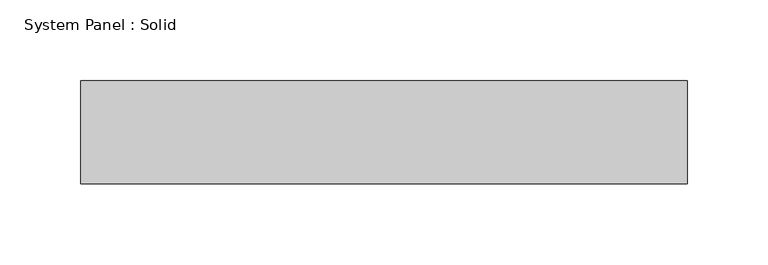
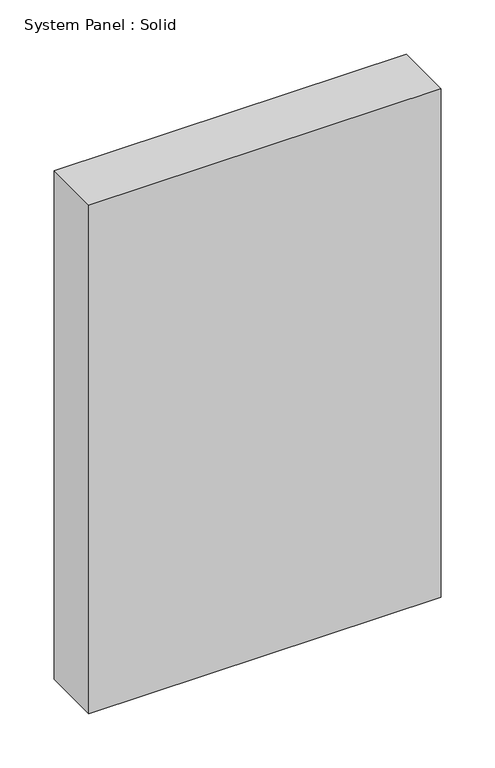
"""IFC4 building model written with IfcOpenShell, lengths in millimetres: plate geometry, System Panel : Solid."""

import ifcopenshell
import ifcopenshell.guid

model = None  # the IFC model being written
_history = None  # IfcOwnerHistory: only IFC2X3 demands one
_inside = {}  # id of a spatial element -> (the spatial element, [elements in it])
_under = {}  # id of a project, library or spatial element -> (it, [spatial elements below it])
_declared = {}  # id of a project -> (the project, [libraries it declares])
_typed = {}  # id of a type object -> (the type object, [elements of that type])
_made_of = {}  # id of a material, layer set ... -> (it, [elements and type objects made of it])


def new_model(schema):
    """Start an empty IFC model of exactly this schema.

    Asked for "IFC4X3", IfcOpenShell would pick the latest addendum, in which some entities
    have other attributes; the version numbers below select the first issue.
    IFC2X3 requires an IfcOwnerHistory on every rooted entity: one is made here for all.
    """
    global model, _history
    if schema == "IFC4X3":
        model = ifcopenshell.file(schema_version=(4, 3, 0, 0))
    else:
        model = ifcopenshell.file(schema=schema)
    _inside.clear()
    _under.clear()
    _declared.clear()
    _typed.clear()
    _made_of.clear()
    _history = None
    if model.schema == "IFC2X3":
        org = make("IfcOrganization", Name="unknown")
        user = make(
            "IfcPersonAndOrganization",
            ThePerson=make("IfcPerson", FamilyName="unknown"),
            TheOrganization=org,
        )
        app = make(
            "IfcApplication",
            ApplicationDeveloper=org,
            Version="unknown",
            ApplicationFullName="unknown",
            ApplicationIdentifier="unknown",
        )
        _history = make(
            "IfcOwnerHistory",
            OwningUser=user,
            OwningApplication=app,
            ChangeAction="ADDED",
            CreationDate=0,
        )
    return model


def make(cls, **values):
    """One entity of the class cls with the attributes given. An attribute that is None is left unset."""
    return model.create_entity(
        cls, **{name: value for name, value in values.items() if value is not None}
    )


def rooted(cls, **values):
    """An entity with a GlobalId (a new one), such as an element, a storey or a relation."""
    return make(cls, GlobalId=ifcopenshell.guid.new(), OwnerHistory=_history, **values)


def si_unit(unit_type, name, prefix=None):
    """IfcSIUnit, for example si_unit("LENGTHUNIT", "METRE", prefix="MILLI")."""
    return make("IfcSIUnit", UnitType=unit_type, Prefix=prefix, Name=name)


def assignment(units):
    """IfcUnitAssignment: the units of a project."""
    return None if units is None else make("IfcUnitAssignment", Units=units)


def point(xyz):
    """IfcCartesianPoint."""
    return None if xyz is None else make("IfcCartesianPoint", Coordinates=xyz)


def direction(xyz):
    """IfcDirection."""
    return None if xyz is None else make("IfcDirection", DirectionRatios=xyz)


def frame(location, z_axis=None, x_axis=None):
    """IfcAxis2Placement3D, a coordinate frame: its origin and axes. An axis left out is left unset."""
    return make(
        "IfcAxis2Placement3D",
        Location=point(location),
        Axis=direction(z_axis),
        RefDirection=direction(x_axis),
    )


def origin():
    """The frame at (0, 0, 0) with its axes left unset."""
    return frame((0.0, 0.0, 0.0))


def origin_with_axes():
    """The frame at (0, 0, 0) with the z axis (0, 0, 1) and the x axis (1, 0, 0) written out."""
    return frame((0.0, 0.0, 0.0), z_axis=(0.0, 0.0, 1.0), x_axis=(1.0, 0.0, 0.0))


def place(relative_to, where):
    """IfcLocalPlacement: puts the frame where relative to a parent placement (None: the world)."""
    return make(
        "IfcLocalPlacement", PlacementRelTo=relative_to, RelativePlacement=where
    )


def context(
    kind, dimensions, precision=None, world=None, true_north=None, identifier=None
):
    """IfcGeometricRepresentationContext, for example the 3D "Model" context."""
    return make(
        "IfcGeometricRepresentationContext",
        ContextIdentifier=identifier,
        ContextType=kind,
        CoordinateSpaceDimension=dimensions,
        Precision=precision,
        WorldCoordinateSystem=world,
        TrueNorth=true_north,
    )


def project(units=None, contexts=None):
    """IfcProject with its units and contexts."""
    return rooted(
        "IfcProject",
        Name="project",
        RepresentationContexts=contexts,
        UnitsInContext=assignment(units),
    )


def spatial(cls, under=None, at=None, **own):
    """A site, building, storey or space (cls), placed at a placement, below another one or the project."""
    s = rooted(cls, ObjectPlacement=at, **own)
    if under is not None:
        _under.setdefault(under.id(), (under, []))[1].append(s)
    return s


def polyline(points):
    """IfcPolyline through the points."""
    return make("IfcPolyline", Points=[point(p) for p in points])


def outline(outer, holes=None, kind="AREA"):
    """IfcArbitraryClosedProfileDef: a profile drawn as a closed curve; with holes, ...WithVoids."""
    if holes is None:
        return make("IfcArbitraryClosedProfileDef", ProfileType=kind, OuterCurve=outer)
    return make(
        "IfcArbitraryProfileDefWithVoids",
        ProfileType=kind,
        OuterCurve=outer,
        InnerCurves=holes,
    )


def extrude(swept, where, along, depth):
    """IfcExtrudedAreaSolid: the profile swept, set in the frame where, extruded along a direction by depth."""
    return make(
        "IfcExtrudedAreaSolid",
        SweptArea=swept,
        Position=where,
        ExtrudedDirection=direction(along),
        Depth=depth,
    )


def shape(context_of_items, identifier, shape_type, items):
    """IfcShapeRepresentation: the items that make up one representation, for example the "Body"."""
    return make(
        "IfcShapeRepresentation",
        ContextOfItems=context_of_items,
        RepresentationIdentifier=identifier,
        RepresentationType=shape_type,
        Items=items,
    )


def source(mapping_origin, context_of_items, identifier, shape_type, items):
    """IfcRepresentationMap: a shape defined once, which mapped items show again and again."""
    return make(
        "IfcRepresentationMap",
        MappingOrigin=mapping_origin,
        MappedRepresentation=shape(context_of_items, identifier, shape_type, items),
    )


def transform(
    local_origin,
    x_axis=None,
    y_axis=None,
    z_axis=None,
    scale=None,
    scale2=None,
    scale3=None,
    uniform=True,
):
    """IfcCartesianTransformationOperator3D, or its non-uniform kind. x_axis, y_axis, z_axis: its Axis1, 2, 3."""
    if uniform:
        return make(
            "IfcCartesianTransformationOperator3D",
            Axis1=direction(x_axis),
            Axis2=direction(y_axis),
            LocalOrigin=point(local_origin),
            Scale=scale,
            Axis3=direction(z_axis),
        )
    return make(
        "IfcCartesianTransformationOperator3DnonUniform",
        Axis1=direction(x_axis),
        Axis2=direction(y_axis),
        LocalOrigin=point(local_origin),
        Scale=scale,
        Axis3=direction(z_axis),
        Scale2=scale2,
        Scale3=scale3,
    )


def mapped(mapping_source, mapping_target):
    """IfcMappedItem: shows the shape of a source again, moved by a transform."""
    return make(
        "IfcMappedItem", MappingSource=mapping_source, MappingTarget=mapping_target
    )


def made_of(thing, what):
    """Note that an element or type object is made of a material, layer set ...; save() writes the relation."""
    if what is not None:
        _made_of.setdefault(what.id(), (what, []))[1].append(thing)
    return thing


def element(
    cls,
    number,
    at=None,
    inside=None,
    cuts=None,
    type_object=None,
    material=None,
    context=None,
    identifier="Body",
    shape_type=None,
    held_by="IfcProductDefinitionShape",
    body=None,
    shapes=None,
    **own,
):
    """One element of the class cls, such as IfcWall. Its Tag is "e" and its number.

    at: its placement. inside: the storey or other place that contains it. cuts: it is an
    opening in that element (IfcRelVoidsElement). A single representation is given by context,
    identifier, shape_type and body (its items); several are given by shapes. held_by: the class
    of the entity that holds the representations. save() writes the other relations.
    """
    e = rooted(cls, Tag="e%d" % number, ObjectPlacement=at, **own)
    if body is not None:
        shapes = [shape(context, identifier, shape_type, body)]
    if shapes is not None:
        e.Representation = make(held_by, Representations=shapes)
    if inside is not None:
        _inside.setdefault(inside.id(), (inside, []))[1].append(e)
    if cuts is not None:
        rooted(
            "IfcRelVoidsElement", RelatingBuildingElement=cuts, RelatedOpeningElement=e
        )
    if type_object is not None:
        _typed.setdefault(type_object.id(), (type_object, []))[1].append(e)
    return made_of(e, material)


def aggregate(whole, parts):
    """IfcRelAggregates: a whole, such as a stair, and the parts it consists of."""
    return rooted("IfcRelAggregates", RelatingObject=whole, RelatedObjects=parts)


def save(model, path):
    """Write the relations noted so far, then the file.

    IfcRelAggregates (storeys below a building ...), IfcRelContainedInSpatialStructure (elements
    in a storey), IfcRelDefinesByType, IfcRelAssociatesMaterial and IfcRelDeclares: one each for
    every whole, place, type object, material and project.
    """
    for whole, parts in _under.values():
        aggregate(whole, parts)
    for where, things in _inside.values():
        rooted(
            "IfcRelContainedInSpatialStructure",
            RelatedElements=things,
            RelatingStructure=where,
        )
    for kind, things in _typed.values():
        rooted("IfcRelDefinesByType", RelatedObjects=things, RelatingType=kind)
    for what, things in _made_of.values():
        rooted("IfcRelAssociatesMaterial", RelatedObjects=things, RelatingMaterial=what)
    for by, libraries in _declared.values():
        rooted("IfcRelDeclares", RelatingContext=by, RelatedDefinitions=libraries)
    model.write(path)


def system_panel_solid_684ff5f5(model_context):
    return source(origin(), model_context, "Body", "SweptSolid", [
        extrude(outline(polyline([(187.3249998, -19.05), (-187.3249998, -19.05), (-187.3249998, 44.45), (187.3249998, 44.45), (187.3249998, -19.05)])), origin_with_axes(), (0.0, 0.0, 1.0), 571.5),
    ])


if __name__ == "__main__":
    model = new_model("IFC4")
    model_context = context("Model", 3, world=origin())
    ifc_project = project(units=[si_unit("LENGTHUNIT", "METRE", prefix="MILLI")], contexts=[model_context])
    site = spatial("IfcSite", under=ifc_project)
    building = spatial("IfcBuilding", under=site)
    placement = place(None, origin())
    system_panel_solid_shape = system_panel_solid_684ff5f5(model_context)
    element("IfcPlate", 1, ObjectType="System Panel : Solid", at=placement, inside=building, context=model_context, shape_type="MappedRepresentation", body=[
        mapped(system_panel_solid_shape, transform((0.0, 0.0, 0.0), x_axis=(1.0, 0.0, 0.0), y_axis=(0.0, 1.0, 0.0), z_axis=(0.0, 0.0, 1.0))),
    ])
    save(model, "model.ifc")

# Revit data of these elements
# Element 1 (IfcPlate, "System Panel : Solid")
#   Materials on its faces: "Default"
# Materials
#   "Default": class "Miscellaneous", colour RGB 127 127 127, transparency 0
